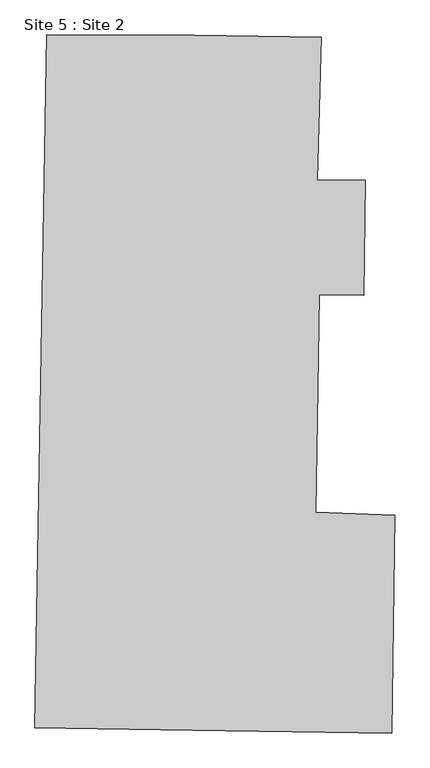
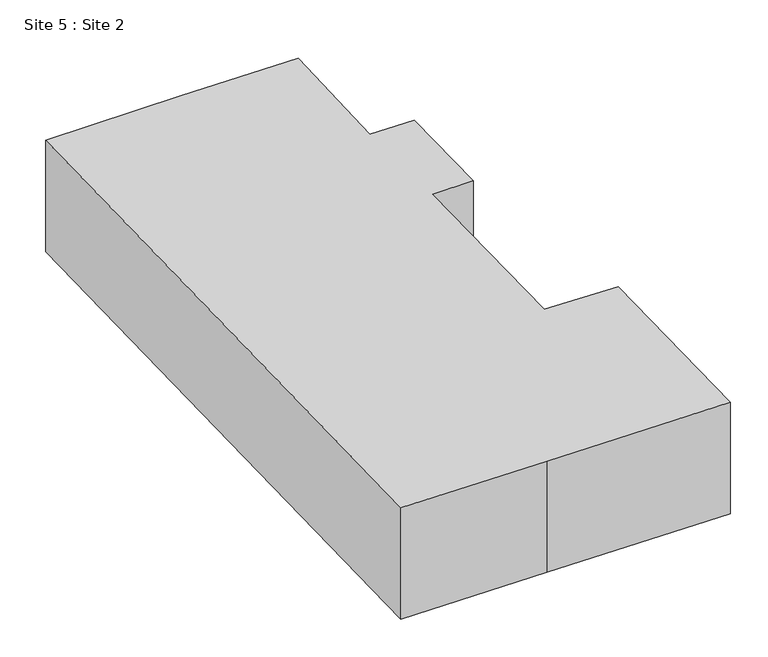
"""IFC4 building model written with IfcOpenShell, lengths in millimetres: geographic element geometry, Site 5 : Site 2."""

import ifcopenshell
import ifcopenshell.guid

model = None  # the IFC model being written
_history = None  # IfcOwnerHistory: only IFC2X3 demands one
_inside = {}  # id of a spatial element -> (the spatial element, [elements in it])
_under = {}  # id of a project, library or spatial element -> (it, [spatial elements below it])
_declared = {}  # id of a project -> (the project, [libraries it declares])
_typed = {}  # id of a type object -> (the type object, [elements of that type])
_made_of = {}  # id of a material, layer set ... -> (it, [elements and type objects made of it])


def new_model(schema):
    """Start an empty IFC model of exactly this schema.

    Asked for "IFC4X3", IfcOpenShell would pick the latest addendum, in which some entities
    have other attributes; the version numbers below select the first issue.
    IFC2X3 requires an IfcOwnerHistory on every rooted entity: one is made here for all.
    """
    global model, _history
    if schema == "IFC4X3":
        model = ifcopenshell.file(schema_version=(4, 3, 0, 0))
    else:
        model = ifcopenshell.file(schema=schema)
    _inside.clear()
    _under.clear()
    _declared.clear()
    _typed.clear()
    _made_of.clear()
    _history = None
    if model.schema == "IFC2X3":
        org = make("IfcOrganization", Name="unknown")
        user = make(
            "IfcPersonAndOrganization",
            ThePerson=make("IfcPerson", FamilyName="unknown"),
            TheOrganization=org,
        )
        app = make(
            "IfcApplication",
            ApplicationDeveloper=org,
            Version="unknown",
            ApplicationFullName="unknown",
            ApplicationIdentifier="unknown",
        )
        _history = make(
            "IfcOwnerHistory",
            OwningUser=user,
            OwningApplication=app,
            ChangeAction="ADDED",
            CreationDate=0,
        )
    return model


def make(cls, **values):
    """One entity of the class cls with the attributes given. An attribute that is None is left unset."""
    return model.create_entity(
        cls, **{name: value for name, value in values.items() if value is not None}
    )


def rooted(cls, **values):
    """An entity with a GlobalId (a new one), such as an element, a storey or a relation."""
    return make(cls, GlobalId=ifcopenshell.guid.new(), OwnerHistory=_history, **values)


def si_unit(unit_type, name, prefix=None):
    """IfcSIUnit, for example si_unit("LENGTHUNIT", "METRE", prefix="MILLI")."""
    return make("IfcSIUnit", UnitType=unit_type, Prefix=prefix, Name=name)


def assignment(units):
    """IfcUnitAssignment: the units of a project."""
    return None if units is None else make("IfcUnitAssignment", Units=units)


def point(xyz):
    """IfcCartesianPoint."""
    return None if xyz is None else make("IfcCartesianPoint", Coordinates=xyz)


def direction(xyz):
    """IfcDirection."""
    return None if xyz is None else make("IfcDirection", DirectionRatios=xyz)


def frame(location, z_axis=None, x_axis=None):
    """IfcAxis2Placement3D, a coordinate frame: its origin and axes. An axis left out is left unset."""
    return make(
        "IfcAxis2Placement3D",
        Location=point(location),
        Axis=direction(z_axis),
        RefDirection=direction(x_axis),
    )


def origin():
    """The frame at (0, 0, 0) with its axes left unset."""
    return frame((0.0, 0.0, 0.0))


def place(relative_to, where):
    """IfcLocalPlacement: puts the frame where relative to a parent placement (None: the world)."""
    return make(
        "IfcLocalPlacement", PlacementRelTo=relative_to, RelativePlacement=where
    )


def context(
    kind, dimensions, precision=None, world=None, true_north=None, identifier=None
):
    """IfcGeometricRepresentationContext, for example the 3D "Model" context."""
    return make(
        "IfcGeometricRepresentationContext",
        ContextIdentifier=identifier,
        ContextType=kind,
        CoordinateSpaceDimension=dimensions,
        Precision=precision,
        WorldCoordinateSystem=world,
        TrueNorth=true_north,
    )


def project(units=None, contexts=None):
    """IfcProject with its units and contexts."""
    return rooted(
        "IfcProject",
        Name="project",
        RepresentationContexts=contexts,
        UnitsInContext=assignment(units),
    )


def spatial(cls, under=None, at=None, **own):
    """A site, building, storey or space (cls), placed at a placement, below another one or the project."""
    s = rooted(cls, ObjectPlacement=at, **own)
    if under is not None:
        _under.setdefault(under.id(), (under, []))[1].append(s)
    return s


def polyline(points):
    """IfcPolyline through the points."""
    return make("IfcPolyline", Points=[point(p) for p in points])


def outline(outer, holes=None, kind="AREA"):
    """IfcArbitraryClosedProfileDef: a profile drawn as a closed curve; with holes, ...WithVoids."""
    if holes is None:
        return make("IfcArbitraryClosedProfileDef", ProfileType=kind, OuterCurve=outer)
    return make(
        "IfcArbitraryProfileDefWithVoids",
        ProfileType=kind,
        OuterCurve=outer,
        InnerCurves=holes,
    )


def extrude(swept, where, along, depth):
    """IfcExtrudedAreaSolid: the profile swept, set in the frame where, extruded along a direction by depth."""
    return make(
        "IfcExtrudedAreaSolid",
        SweptArea=swept,
        Position=where,
        ExtrudedDirection=direction(along),
        Depth=depth,
    )


def shape(context_of_items, identifier, shape_type, items):
    """IfcShapeRepresentation: the items that make up one representation, for example the "Body"."""
    return make(
        "IfcShapeRepresentation",
        ContextOfItems=context_of_items,
        RepresentationIdentifier=identifier,
        RepresentationType=shape_type,
        Items=items,
    )


def source(mapping_origin, context_of_items, identifier, shape_type, items):
    """IfcRepresentationMap: a shape defined once, which mapped items show again and again."""
    return make(
        "IfcRepresentationMap",
        MappingOrigin=mapping_origin,
        MappedRepresentation=shape(context_of_items, identifier, shape_type, items),
    )


def transform(
    local_origin,
    x_axis=None,
    y_axis=None,
    z_axis=None,
    scale=None,
    scale2=None,
    scale3=None,
    uniform=True,
):
    """IfcCartesianTransformationOperator3D, or its non-uniform kind. x_axis, y_axis, z_axis: its Axis1, 2, 3."""
    if uniform:
        return make(
            "IfcCartesianTransformationOperator3D",
            Axis1=direction(x_axis),
            Axis2=direction(y_axis),
            LocalOrigin=point(local_origin),
            Scale=scale,
            Axis3=direction(z_axis),
        )
    return make(
        "IfcCartesianTransformationOperator3DnonUniform",
        Axis1=direction(x_axis),
        Axis2=direction(y_axis),
        LocalOrigin=point(local_origin),
        Scale=scale,
        Axis3=direction(z_axis),
        Scale2=scale2,
        Scale3=scale3,
    )


def mapped(mapping_source, mapping_target):
    """IfcMappedItem: shows the shape of a source again, moved by a transform."""
    return make(
        "IfcMappedItem", MappingSource=mapping_source, MappingTarget=mapping_target
    )


def made_of(thing, what):
    """Note that an element or type object is made of a material, layer set ...; save() writes the relation."""
    if what is not None:
        _made_of.setdefault(what.id(), (what, []))[1].append(thing)
    return thing


def element(
    cls,
    number,
    at=None,
    inside=None,
    cuts=None,
    type_object=None,
    material=None,
    context=None,
    identifier="Body",
    shape_type=None,
    held_by="IfcProductDefinitionShape",
    body=None,
    shapes=None,
    **own,
):
    """One element of the class cls, such as IfcWall. Its Tag is "e" and its number.

    at: its placement. inside: the storey or other place that contains it. cuts: it is an
    opening in that element (IfcRelVoidsElement). A single representation is given by context,
    identifier, shape_type and body (its items); several are given by shapes. held_by: the class
    of the entity that holds the representations. save() writes the other relations.
    """
    e = rooted(cls, Tag="e%d" % number, ObjectPlacement=at, **own)
    if body is not None:
        shapes = [shape(context, identifier, shape_type, body)]
    if shapes is not None:
        e.Representation = make(held_by, Representations=shapes)
    if inside is not None:
        _inside.setdefault(inside.id(), (inside, []))[1].append(e)
    if cuts is not None:
        rooted(
            "IfcRelVoidsElement", RelatingBuildingElement=cuts, RelatedOpeningElement=e
        )
    if type_object is not None:
        _typed.setdefault(type_object.id(), (type_object, []))[1].append(e)
    return made_of(e, material)


def aggregate(whole, parts):
    """IfcRelAggregates: a whole, such as a stair, and the parts it consists of."""
    return rooted("IfcRelAggregates", RelatingObject=whole, RelatedObjects=parts)


def save(model, path):
    """Write the relations noted so far, then the file.

    IfcRelAggregates (storeys below a building ...), IfcRelContainedInSpatialStructure (elements
    in a storey), IfcRelDefinesByType, IfcRelAssociatesMaterial and IfcRelDeclares: one each for
    every whole, place, type object, material and project.
    """
    for whole, parts in _under.values():
        aggregate(whole, parts)
    for where, things in _inside.values():
        rooted(
            "IfcRelContainedInSpatialStructure",
            RelatedElements=things,
            RelatingStructure=where,
        )
    for kind, things in _typed.values():
        rooted("IfcRelDefinesByType", RelatedObjects=things, RelatingType=kind)
    for what, things in _made_of.values():
        rooted("IfcRelAssociatesMaterial", RelatedObjects=things, RelatingMaterial=what)
    for by, libraries in _declared.values():
        rooted("IfcRelDeclares", RelatingContext=by, RelatedDefinitions=libraries)
    model.write(path)


def site_5_site_2_326ef9a9(model_context):
    return source(origin(), model_context, "Body", "SweptSolid", [
        extrude(outline(polyline([(8729.3511309, 115761.4537123), (8505.6065901, 107331.1517319), (11350.1096011, 107289.9427165), (11251.503902, 100483.5629679), (8610.1793752, 100521.8284866), (8423.2700009, 87620.1788693), (13094.9076516, 87450.8912577), (12907.9988905, 74549.2839684), (1123.6383438, 74720.0069008), (-8222.5803931, 74855.4078726), (-7526.4162506, 115895.3465696), (1211.7387515, 115870.3632136), (8729.3511309, 115761.4537123)])), frame((0.0, 0.0, 266395.2), z_axis=(0.0, 0.0, 1.0), x_axis=(1.0, 0.0, 0.0)), (0.0, 0.0, 1.0), 7620.0),
    ])


if __name__ == "__main__":
    model = new_model("IFC4")
    model_context = context("Model", 3, world=origin())
    ifc_project = project(units=[si_unit("LENGTHUNIT", "METRE", prefix="MILLI")], contexts=[model_context])
    site = spatial("IfcSite", under=ifc_project)
    building = spatial("IfcBuilding", under=site)
    placement = place(None, origin())
    site_5_site_2_shape = site_5_site_2_326ef9a9(model_context)
    element("IfcGeographicElement", 1, ObjectType="Site 5 : Site 2", at=placement, inside=building, context=model_context, shape_type="MappedRepresentation", body=[
        mapped(site_5_site_2_shape, transform((0.0, 0.0, 0.0), x_axis=(1.0, 0.0, 0.0), y_axis=(0.0, 1.0, 0.0), z_axis=(0.0, 0.0, 1.0))),
    ])
    save(model, "model.ifc")

# Revit data of these elements
# Element 1 (IfcGeographicElement, "Site 5 : Site 2")
#   Materials on its faces: "EXISTING BUILDING"
# Materials
#   "EXISTING BUILDING": class "Generic", colour RGB 120 120 120, transparency 0, Cost = 0
